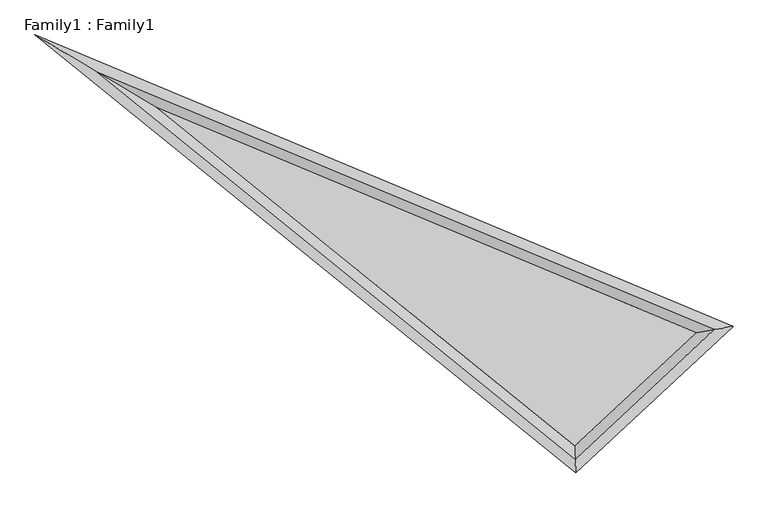
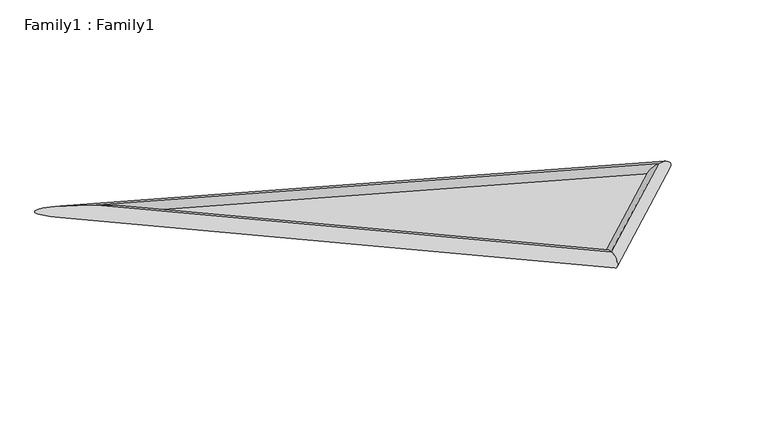
"""IFC4 building model written with IfcOpenShell, lengths in millimetres: proxy geometry, Family1 : Family1."""

from ifc_helpers import new_model, si_unit, frame, origin, origin_with_axes, place, context, project, spatial, polyline, ellipse_curve, outline, extrude, source, transform, mapped, element, save
from ifc_brep_helpers import cylinder_surface, advanced_brep


def family1_family1_134ea19e(model_context):
    return source(origin(), model_context, "Body", "SolidModel", [
        extrude(outline(polyline([(2013.7308019, -1203.5740312), (-2604.7087242, 2539.0469192), (3357.9003733, 48.4683169), (2013.7308019, -1203.5740312)])), origin_with_axes(), (0.0, 0.0, 1.0), 34.1328789),
        advanced_brep(
        [(2013.7308019, -1203.5740312, 100.0), (2013.7308019, -1203.5740312, -100.0), (-2604.7087242, 2539.0469192, -100.0), (-2604.7087242, 2539.0469192, 100.0), (3357.9003733, 48.4683169, -100.0), (3357.9003733, 48.4683169, 100.0)],
        [
            (0, 1, ellipse_curve(frame((2013.7308019, -1203.5740312, 0.0), z_axis=(-0.9994066795498644, -0.034442544492450995, 0.0), x_axis=(0.03444254449245123, -0.9994066795498646, 0.0)), 132.4890283, 100.0)),
            (1, 2),
            (2, 3, ellipse_curve(frame((-2604.7087242, 2539.0469192, 0.0), z_axis=(-0.5127200273078839, -0.8585558651581171, 0.0), x_axis=(0.8585558651581171, -0.5127200273078838, 0.0)), 703.2569664, 100.0)),
            (3, 0),
            (1, 0, ellipse_curve(frame((2013.7308019, -1203.5740312, 0.0), z_axis=(-0.9994066795498644, -0.034442544492450995, 0.0), x_axis=(0.03444254449245123, -0.9994066795498646, 0.0)), 132.4890283, 100.0)),
            (3, 2, ellipse_curve(frame((-2604.7087242, 2539.0469192, 0.0), z_axis=(-0.5127200273078839, -0.8585558651581171, 0.0), x_axis=(0.8585558651581171, -0.5127200273078838, 0.0)), 703.2569664, 100.0)),
            (2, 4),
            (4, 5, ellipse_curve(frame((3357.9003733, 48.4683169, 0.0), z_axis=(-0.17620372625746822, 0.9843537203937329, 0.0), x_axis=(-0.9843537203937328, -0.17620372625746825, 0.0)), 184.5063833, 100.0)),
            (5, 3),
            (5, 4, ellipse_curve(frame((3357.9003733, 48.4683169, 0.0), z_axis=(-0.17620372625746822, 0.9843537203937329, 0.0), x_axis=(-0.9843537203937328, -0.17620372625746825, 0.0)), 184.5063833, 100.0)),
            (4, 1),
            (0, 5),
        ],
        [
            cylinder_surface(frame((2013.7308019, -1203.5740312, 0.0), z_axis=(0.7769252270225571, -0.6295928776725069, 0.0), x_axis=(-0.6295928776725069, -0.7769252270225571, 0.0)), 100.0),
            cylinder_surface(frame((-2604.7087242, 2539.0469192, 0.0), z_axis=(-0.9227382233503376, 0.3854272579466354, 0.0), x_axis=(0.3854272579466354, 0.9227382233503376, 0.0)), 100.0),
            cylinder_surface(frame((3357.9003733, 48.4683169, 0.0), z_axis=(0.7317380821665097, 0.6815859293642134, 0.0), x_axis=(0.6815859293642134, -0.7317380821665097, 0.0)), 100.0),
        ],
        [
            (0, [[1, 2, 3, 4]]),
            (0, [[5, -4, 6, -2]]),
            (1, [[-3, 7, 8, 9]]),
            (1, [[-6, -9, 10, -7]]),
            (2, [[-8, 11, -1, 12]]),
            (2, [[-10, -12, -5, -11]]),
        ],
    ),
    ])


if __name__ == "__main__":
    model = new_model("IFC4")
    model_context = context("Model", 3, world=origin())
    ifc_project = project(units=[si_unit("LENGTHUNIT", "METRE", prefix="MILLI")], contexts=[model_context])
    site = spatial("IfcSite", under=ifc_project)
    building = spatial("IfcBuilding", under=site)
    placement = place(None, origin())
    family1_family1_shape = family1_family1_134ea19e(model_context)
    element("IfcBuildingElementProxy", 1, Name="Family1 : Family1", ObjectType="Family1 : Family1", at=placement, inside=building, context=model_context, shape_type="MappedRepresentation", body=[
        mapped(family1_family1_shape, transform((0.0, 0.0, 0.0), x_axis=(1.0, 0.0, 0.0), y_axis=(0.0, 1.0, 0.0), z_axis=(0.0, 0.0, 1.0))),
    ])
    save(model, "model.ifc")

# Revit data of these elements
# Type "Family1 : Family1"
#   Default Elevation = 0
# Element 1 (IfcBuildingElementProxy, "Family1 : Family1")
#   Materials on its faces: "Glass"
# Materials
#   "Glass": class "Glass", colour RGB 0 128 192, transparency 0.9, Description = "Soda Lime Glass", Cost = 0
